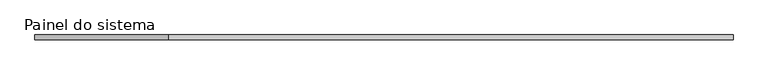
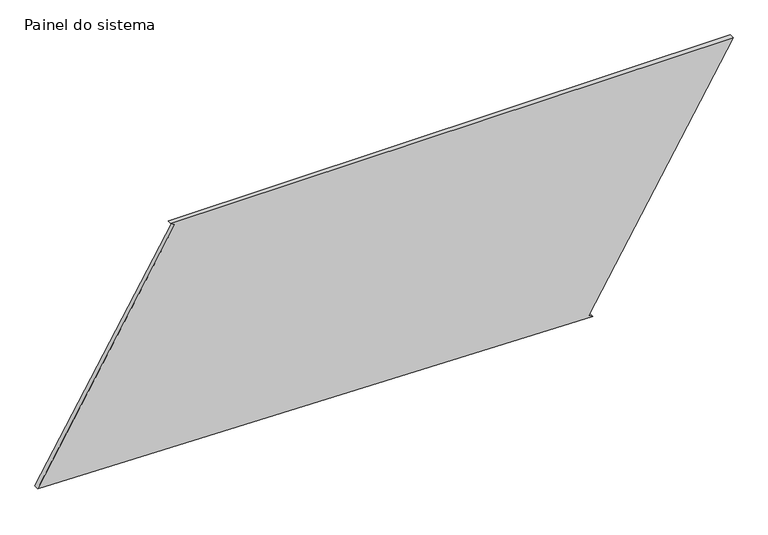
"""IFC4 building model written with IfcOpenShell, lengths in millimetres: plate geometry, Painel do sistema : Envidraçado."""

from ifc_helpers import new_model, si_unit, frame, origin, place, context, project, spatial, polyline, outline, extrude, source, transform, mapped, element, save


def painel_do_sistema_94b568e9(model_context):
    return source(origin(), model_context, "Body", "SweptSolid", [
        extrude(outline(polyline([(0.0, 1092.5400208), (12.7505939, 1071.036013), (1295.6559034, 1831.7223363), (1295.6559034, -1130.0847777), (1282.9053094, -1108.5807698), (63.3196186, -1831.7223363), (0.0, 1092.5400208)])), frame((0.0, 24.5, 0.0), z_axis=(0.0, 1.0, 0.0), x_axis=(0.0, 0.0, 1.0)), (0.0, 0.0, 1.0), 25.0),
    ])


if __name__ == "__main__":
    model = new_model("IFC4")
    model_context = context("Model", 3, world=origin())
    ifc_project = project(units=[si_unit("LENGTHUNIT", "METRE", prefix="MILLI")], contexts=[model_context])
    site = spatial("IfcSite", under=ifc_project)
    building = spatial("IfcBuilding", under=site)
    placement = place(None, origin())
    painel_do_sistema_shape = painel_do_sistema_94b568e9(model_context)
    element("IfcPlate", 1, ObjectType="Painel do sistema : Envidraçado", at=placement, inside=building, context=model_context, shape_type="MappedRepresentation", body=[
        mapped(painel_do_sistema_shape, transform((0.0, 0.0, 0.0), x_axis=(1.0, 0.0, 0.0), y_axis=(0.0, 1.0, 0.0), z_axis=(0.0, 0.0, 1.0))),
    ])
    save(model, "model.ifc")

# Revit data of these elements
# Type "Painel do sistema : Envidraçado"
#   Construction Type Id = "GSP4R"
#   Analytic Construction = "Vidraça única Pilkington 1/8 pol"
#   Visual Light Transmittance = 0.9
#   Solar Heat Gain Coefficient = 0.86
#   Heat Transfer Coefficient (U) = 6.7069 W/(m²·K)
# Element 1 (IfcPlate, "Painel do sistema : Envidraçado")
#   Materials on its faces: "Vidro"
# Materials
#   "Vidro": class "Vidro", colour RGB 0 128 192, transparency 0.9, Description = "Vidro de sílica", Cost = 0
